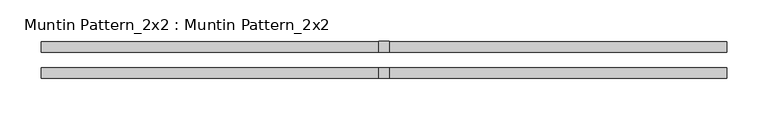
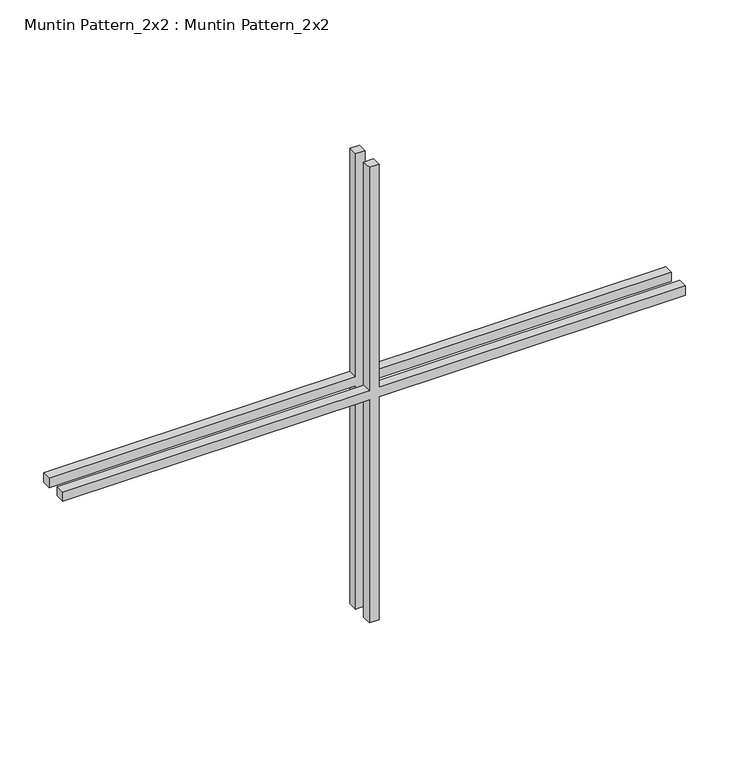
"""IFC4 building model written with IfcOpenShell, lengths in millimetres: proxy geometry, Muntin Pattern_2x2 : Muntin Pattern_2x2."""

from ifc_helpers import new_model, si_unit, frame, origin, place, context, project, spatial, polyline, outline, extrude, source, transform, mapped, element, save


def muntin_pattern_2x2_muntin_pattern_2x2_9cade0ad(model_context):
    return source(origin(), model_context, "Body", "SweptSolid", [
        extrude(outline(polyline([(325.4375, -6.35), (325.4375, -412.75), (312.7375, -412.75), (312.7375, -6.35), (0.0, -6.35), (0.0, 6.35), (312.7375, 6.35), (312.7375, 412.75), (325.4375, 412.75), (325.4375, 6.35), (638.175, 6.35), (638.175, -6.35), (325.4375, -6.35)])), frame((0.0, -22.225, 0.0), z_axis=(0.0, 1.0, 0.0), x_axis=(0.0, 0.0, 1.0)), (0.0, 0.0, 1.0), 12.7),
        extrude(outline(polyline([(325.4375, -6.35), (325.4375, -412.75), (312.7375, -412.75), (312.7375, -6.35), (0.0, -6.35), (0.0, 6.35), (312.7375, 6.35), (312.7375, 412.75), (325.4375, 412.75), (325.4375, 6.35), (638.175, 6.35), (638.175, -6.35), (325.4375, -6.35)])), frame((0.0, 9.525, 0.0), z_axis=(0.0, 1.0, 0.0), x_axis=(0.0, 0.0, 1.0)), (0.0, 0.0, 1.0), 12.7),
    ])


if __name__ == "__main__":
    model = new_model("IFC4")
    model_context = context("Model", 3, world=origin())
    ifc_project = project(units=[si_unit("LENGTHUNIT", "METRE", prefix="MILLI")], contexts=[model_context])
    site = spatial("IfcSite", under=ifc_project)
    building = spatial("IfcBuilding", under=site)
    placement = place(None, origin())
    muntin_pattern_2x2_muntin_pattern_2x2_shape = muntin_pattern_2x2_muntin_pattern_2x2_9cade0ad(model_context)
    element("IfcBuildingElementProxy", 1, Name="Muntin Pattern_2x2 : Muntin Pattern_2x2", ObjectType="Muntin Pattern_2x2 : Muntin Pattern_2x2", at=placement, inside=building, context=model_context, shape_type="MappedRepresentation", body=[
        mapped(muntin_pattern_2x2_muntin_pattern_2x2_shape, transform((0.0, 0.0, 0.0), x_axis=(1.0, 0.0, 0.0), y_axis=(0.0, 1.0, 0.0), z_axis=(0.0, 0.0, 1.0))),
    ])
    save(model, "model.ifc")

# Revit data of these elements
# Type "Muntin Pattern_2x2 : Muntin Pattern_2x2"
#   Width [instance default] = 4' - 0"
#   Thickness = 0' - 0 1/2"
#   Height [instance default] = 4' - 0"
#   Distance = 0' - 0 3/4"
#   Interior Material [instance default] = none
#   Exterior Material [instance default] = none
# Element 1 (IfcBuildingElementProxy, "Muntin Pattern_2x2 : Muntin Pattern_2x2")
#   Width = 2' - 8 1/2"
#   Height = 2' - 1 1/8"
#   Interior Material = Wood - Stained
#   Exterior Material = Clad - White
#   Materials on its faces: "Clad - White", "Wood - Stained"
# Materials
#   "Clad - White": class "Wood", colour RGB 242 242 238, transparency 0, Cost = 0
#   "Wood - Stained": class "Wood", colour RGB 224 178 126, transparency 0, Cost = 0
